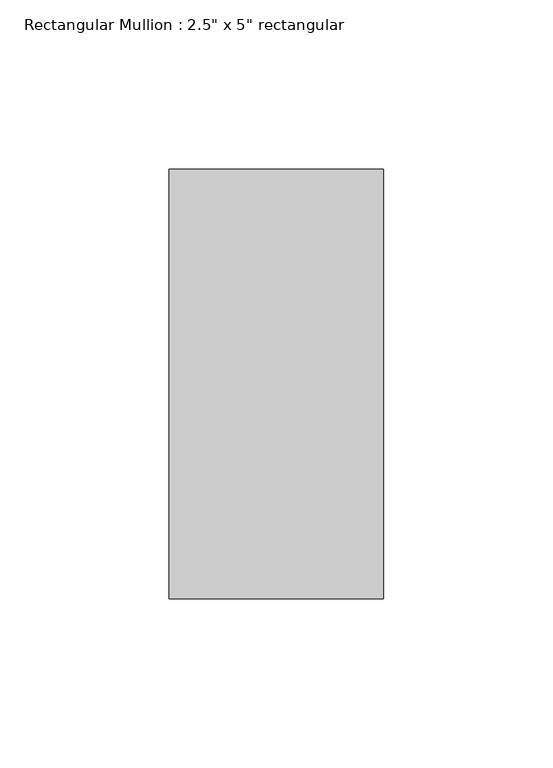
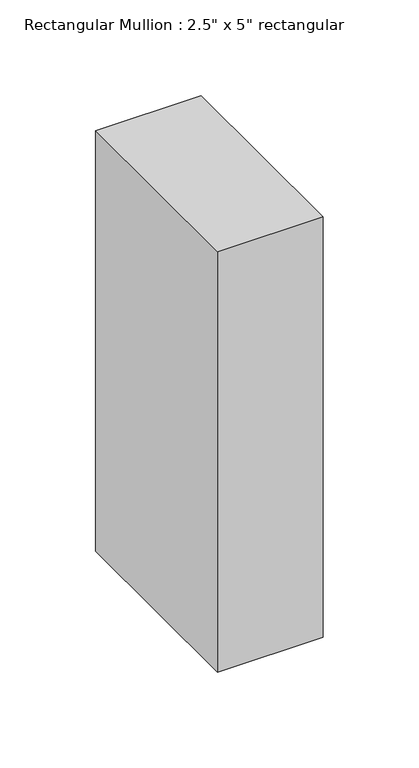
"""IFC4 building model written with IfcOpenShell, lengths in millimetres: member geometry."""

from ifc_helpers import new_model, si_unit, frame, origin, place, context, project, spatial, polyline, outline, extrude, source, transform, mapped, element, save


def member_40e8ea34(model_context):
    return source(origin(), model_context, "Body", "SweptSolid", [
        extrude(outline(polyline([(31.75, 63.5), (31.75, -63.5), (-31.75, -63.5), (-31.75, 63.5), (31.75, 63.5)])), frame((0.0, 0.0, -267.49375), z_axis=(0.0, 0.0, 1.0), x_axis=(1.0, 0.0, 0.0)), (0.0, 0.0, 1.0), 267.49375),
    ])


if __name__ == "__main__":
    model = new_model("IFC4")
    model_context = context("Model", 3, world=origin())
    ifc_project = project(units=[si_unit("LENGTHUNIT", "METRE", prefix="MILLI")], contexts=[model_context])
    site = spatial("IfcSite", under=ifc_project)
    building = spatial("IfcBuilding", under=site)
    placement = place(None, origin())
    member_shape = member_40e8ea34(model_context)
    element("IfcMember", 1, ObjectType="Rectangular Mullion : 2.5\" x 5\" rectangular", at=placement, inside=building, context=model_context, shape_type="MappedRepresentation", body=[
        mapped(member_shape, transform((0.0, 0.0, 0.0), x_axis=(1.0, 0.0, 0.0), y_axis=(0.0, 1.0, 0.0), z_axis=(0.0, 0.0, 1.0))),
    ])
    save(model, "model.ifc")

# Revit data of these elements
# Type "Rectangular Mullion : 2.5\" x 5\" rectangular"
#   built-in parameter 1007304 = 0.416667 (stored number, unit not read)
#   built-in parameter 1007301 = 0.104167 (stored number, unit not read)
#   built-in parameter 1007300 = 0.104167 (stored number, unit not read)
# Element 1 (IfcMember, "Rectangular Mullion : 2.5\" x 5\" rectangular")
#   Materials on its faces: "Metal - Aluminum"
# Materials
#   "Metal - Aluminum": class "Metal", colour RGB 140 140 140, transparency 0
